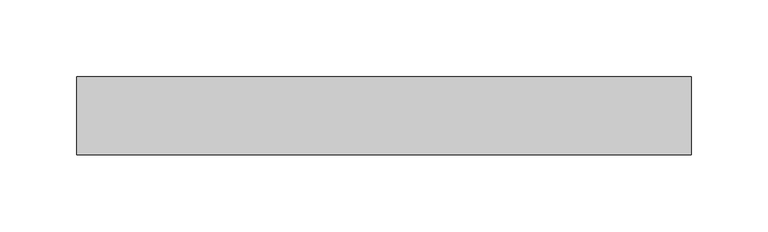
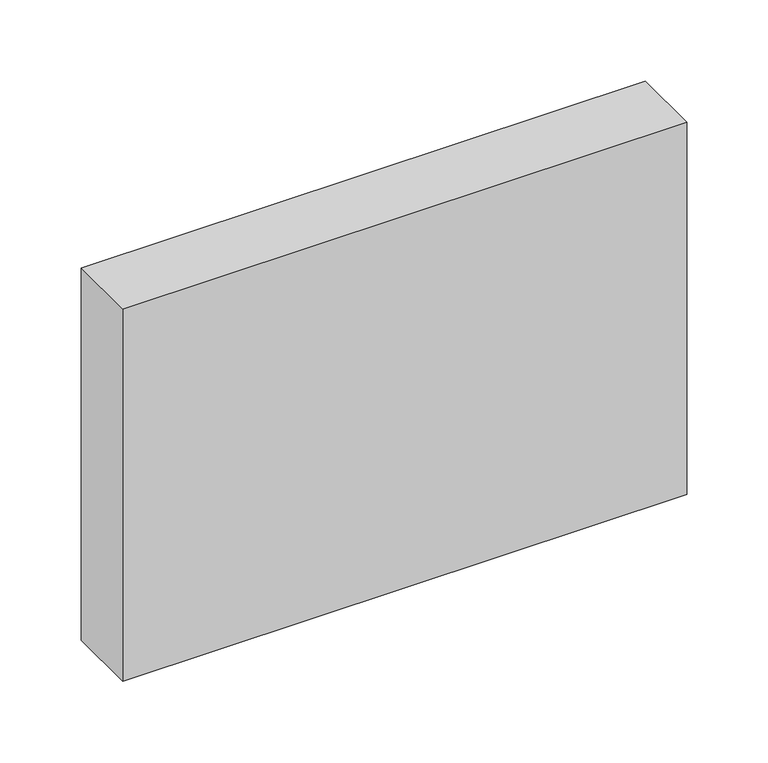
"""IFC4 building model written with IfcOpenShell, lengths in millimetres: proxy geometry, Seqm-Seat Cover Disp-UH-3D : Seqm-Seat Cover Disp-UH-3D."""

from ifc_helpers import new_model, si_unit, frame, origin, place, context, project, spatial, polyline, outline, extrude, source, transform, mapped, element, save


def specialty_equipment_f409795c(model_context):
    return source(origin(), model_context, "Body", "SweptSolid", [
        extrude(outline(polyline([(200.025, 0.0), (200.025, -50.8), (-200.025, -50.8), (-200.025, 0.0), (200.025, 0.0)])), frame((0.0, 0.0, 939.8), z_axis=(0.0, 0.0, 1.0), x_axis=(1.0, 0.0, 0.0)), (0.0, 0.0, 1.0), 279.4),
    ])


if __name__ == "__main__":
    model = new_model("IFC4")
    model_context = context("Model", 3, world=origin())
    ifc_project = project(units=[si_unit("LENGTHUNIT", "METRE", prefix="MILLI")], contexts=[model_context])
    site = spatial("IfcSite", under=ifc_project)
    building = spatial("IfcBuilding", under=site)
    placement = place(None, origin())
    specialty_equipment_shape = specialty_equipment_f409795c(model_context)
    element("IfcBuildingElementProxy", 1, Name="Seqm-Seat Cover Disp-UH-3D : Seqm-Seat Cover Disp-UH-3D", ObjectType="Seqm-Seat Cover Disp-UH-3D : Seqm-Seat Cover Disp-UH-3D", at=placement, inside=building, context=model_context, shape_type="MappedRepresentation", body=[
        mapped(specialty_equipment_shape, transform((0.0, 0.0, 0.0), x_axis=(1.0, 0.0, 0.0), y_axis=(0.0, 1.0, 0.0), z_axis=(0.0, 0.0, 1.0))),
    ])
    save(model, "model.ifc")

# Revit data of these elements
# Type "Seqm-Seat Cover Disp-UH-3D : Seqm-Seat Cover Disp-UH-3D"
#   Width = 1' - 3 3/4"
#   Height from Floor = 3' - 1"
#   Height = 0' - 11"
#   Depth = 0' - 2"
